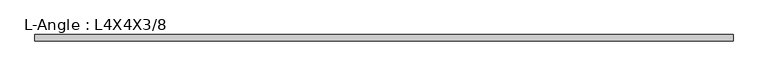
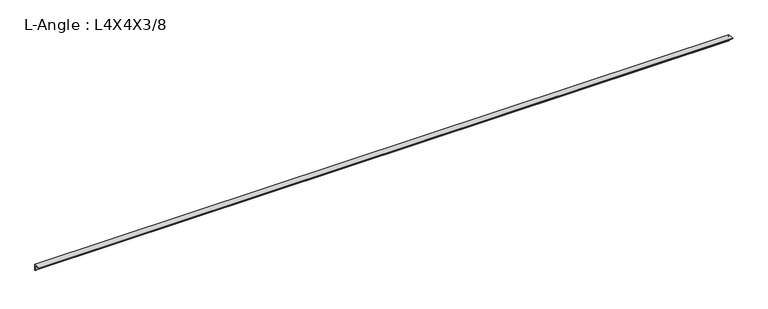
"""IFC4 building model written with IfcOpenShell, lengths in millimetres: beam geometry, L-Angle : L4X4X3/8."""

from ifc_helpers import new_model, si_unit, point, frame, frame_2d, origin, place, context, project, spatial, polyline, circle_curve, trimmed, segment, composite_curve, outline, extrude, source, transform, mapped, element, save


def l_angle_l4x4x3_8_dd29d48c(model_context):
    return source(origin(), model_context, "Body", "SweptSolid", [
        extrude(outline(composite_curve([segment(polyline([(28.702, 28.702), (28.702, -72.898)]), True, "CONTINUOUS"), segment(trimmed(circle_curve(frame_2d((28.702, -63.373)), 9.525), [point((28.702, -72.898))], [point((19.177, -63.373))], False, "CARTESIAN"), True, "CONTINUOUS"), segment(polyline([(19.177, -63.373), (19.177, 9.652)]), True, "CONTINUOUS"), segment(trimmed(circle_curve(frame_2d((9.652, 9.652)), 9.525), [point((19.177, 9.652))], [point((9.652, 19.177))], True, "CARTESIAN"), True, "CONTINUOUS"), segment(polyline([(9.652, 19.177), (-63.373, 19.177)]), True, "CONTINUOUS"), segment(trimmed(circle_curve(frame_2d((-63.373, 28.702)), 9.525), [point((-63.373, 19.177))], [point((-72.898, 28.702))], False, "CARTESIAN"), True, "CONTINUOUS"), segment(polyline([(-72.898, 28.702), (28.702, 28.702)]), True, "CONTINUOUS")], self_intersect=False)), frame((-5651.5, 0.0, 0.0), z_axis=(1.0, 0.0, 0.0), x_axis=(0.0, 1.0, 0.0)), (0.0, 0.0, 1.0), 11303.0),
    ])


if __name__ == "__main__":
    model = new_model("IFC4")
    model_context = context("Model", 3, world=origin())
    ifc_project = project(units=[si_unit("LENGTHUNIT", "METRE", prefix="MILLI")], contexts=[model_context])
    site = spatial("IfcSite", under=ifc_project)
    building = spatial("IfcBuilding", under=site)
    placement = place(None, origin())
    l_angle_l4x4x3_8_shape = l_angle_l4x4x3_8_dd29d48c(model_context)
    element("IfcBeam", 1, ObjectType="L-Angle : L4X4X3/8", at=placement, inside=building, context=model_context, shape_type="MappedRepresentation", body=[
        mapped(l_angle_l4x4x3_8_shape, transform((0.0, 0.0, 0.0), x_axis=(1.0, 0.0, 0.0), y_axis=(0.0, 1.0, 0.0), z_axis=(0.0, 0.0, 1.0))),
    ])
    save(model, "model.ifc")

# Revit data of these elements
# Type "L-Angle : L4X4X3/8"
#   Assembly Code = "B10"
#   k = 0' - 0 3/4"
#   W = 9.8
#   Length [instance default] = 5' - 0"
#   b = 0' - 4"
#   d = 0' - 4"
#   t = 0' - 0 3/8"
#   x = 0' - 1.13"
#   y = 0' - 1.13"
#   A = 0.0198611 SF
#   Structural Material [instance default] = Steel ASTM A36
# Element 1 (IfcBeam, "L-Angle : L4X4X3/8")
#   Materials on its faces: "Steel ASTM A36"
# Materials
#   "Steel ASTM A36": class "Metal", colour RGB 199 199 199, transparency 0, Description = "Structural steel, ASTM A36 Grade B, mill finish", Cost = 0
